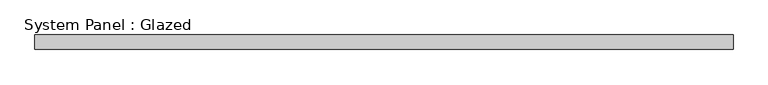
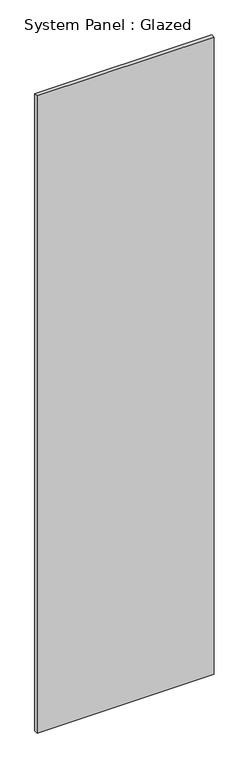
"""IFC4 building model written with IfcOpenShell, lengths in millimetres: plate geometry, System Panel : Glazed."""

import ifcopenshell
import ifcopenshell.guid

model = None  # the IFC model being written
_history = None  # IfcOwnerHistory: only IFC2X3 demands one
_inside = {}  # id of a spatial element -> (the spatial element, [elements in it])
_under = {}  # id of a project, library or spatial element -> (it, [spatial elements below it])
_declared = {}  # id of a project -> (the project, [libraries it declares])
_typed = {}  # id of a type object -> (the type object, [elements of that type])
_made_of = {}  # id of a material, layer set ... -> (it, [elements and type objects made of it])


def new_model(schema):
    """Start an empty IFC model of exactly this schema.

    Asked for "IFC4X3", IfcOpenShell would pick the latest addendum, in which some entities
    have other attributes; the version numbers below select the first issue.
    IFC2X3 requires an IfcOwnerHistory on every rooted entity: one is made here for all.
    """
    global model, _history
    if schema == "IFC4X3":
        model = ifcopenshell.file(schema_version=(4, 3, 0, 0))
    else:
        model = ifcopenshell.file(schema=schema)
    _inside.clear()
    _under.clear()
    _declared.clear()
    _typed.clear()
    _made_of.clear()
    _history = None
    if model.schema == "IFC2X3":
        org = make("IfcOrganization", Name="unknown")
        user = make(
            "IfcPersonAndOrganization",
            ThePerson=make("IfcPerson", FamilyName="unknown"),
            TheOrganization=org,
        )
        app = make(
            "IfcApplication",
            ApplicationDeveloper=org,
            Version="unknown",
            ApplicationFullName="unknown",
            ApplicationIdentifier="unknown",
        )
        _history = make(
            "IfcOwnerHistory",
            OwningUser=user,
            OwningApplication=app,
            ChangeAction="ADDED",
            CreationDate=0,
        )
    return model


def make(cls, **values):
    """One entity of the class cls with the attributes given. An attribute that is None is left unset."""
    return model.create_entity(
        cls, **{name: value for name, value in values.items() if value is not None}
    )


def rooted(cls, **values):
    """An entity with a GlobalId (a new one), such as an element, a storey or a relation."""
    return make(cls, GlobalId=ifcopenshell.guid.new(), OwnerHistory=_history, **values)


def si_unit(unit_type, name, prefix=None):
    """IfcSIUnit, for example si_unit("LENGTHUNIT", "METRE", prefix="MILLI")."""
    return make("IfcSIUnit", UnitType=unit_type, Prefix=prefix, Name=name)


def assignment(units):
    """IfcUnitAssignment: the units of a project."""
    return None if units is None else make("IfcUnitAssignment", Units=units)


def point(xyz):
    """IfcCartesianPoint."""
    return None if xyz is None else make("IfcCartesianPoint", Coordinates=xyz)


def direction(xyz):
    """IfcDirection."""
    return None if xyz is None else make("IfcDirection", DirectionRatios=xyz)


def frame(location, z_axis=None, x_axis=None):
    """IfcAxis2Placement3D, a coordinate frame: its origin and axes. An axis left out is left unset."""
    return make(
        "IfcAxis2Placement3D",
        Location=point(location),
        Axis=direction(z_axis),
        RefDirection=direction(x_axis),
    )


def origin():
    """The frame at (0, 0, 0) with its axes left unset."""
    return frame((0.0, 0.0, 0.0))


def origin_with_axes():
    """The frame at (0, 0, 0) with the z axis (0, 0, 1) and the x axis (1, 0, 0) written out."""
    return frame((0.0, 0.0, 0.0), z_axis=(0.0, 0.0, 1.0), x_axis=(1.0, 0.0, 0.0))


def place(relative_to, where):
    """IfcLocalPlacement: puts the frame where relative to a parent placement (None: the world)."""
    return make(
        "IfcLocalPlacement", PlacementRelTo=relative_to, RelativePlacement=where
    )


def context(
    kind, dimensions, precision=None, world=None, true_north=None, identifier=None
):
    """IfcGeometricRepresentationContext, for example the 3D "Model" context."""
    return make(
        "IfcGeometricRepresentationContext",
        ContextIdentifier=identifier,
        ContextType=kind,
        CoordinateSpaceDimension=dimensions,
        Precision=precision,
        WorldCoordinateSystem=world,
        TrueNorth=true_north,
    )


def project(units=None, contexts=None):
    """IfcProject with its units and contexts."""
    return rooted(
        "IfcProject",
        Name="project",
        RepresentationContexts=contexts,
        UnitsInContext=assignment(units),
    )


def spatial(cls, under=None, at=None, **own):
    """A site, building, storey or space (cls), placed at a placement, below another one or the project."""
    s = rooted(cls, ObjectPlacement=at, **own)
    if under is not None:
        _under.setdefault(under.id(), (under, []))[1].append(s)
    return s


def polyline(points):
    """IfcPolyline through the points."""
    return make("IfcPolyline", Points=[point(p) for p in points])


def outline(outer, holes=None, kind="AREA"):
    """IfcArbitraryClosedProfileDef: a profile drawn as a closed curve; with holes, ...WithVoids."""
    if holes is None:
        return make("IfcArbitraryClosedProfileDef", ProfileType=kind, OuterCurve=outer)
    return make(
        "IfcArbitraryProfileDefWithVoids",
        ProfileType=kind,
        OuterCurve=outer,
        InnerCurves=holes,
    )


def extrude(swept, where, along, depth):
    """IfcExtrudedAreaSolid: the profile swept, set in the frame where, extruded along a direction by depth."""
    return make(
        "IfcExtrudedAreaSolid",
        SweptArea=swept,
        Position=where,
        ExtrudedDirection=direction(along),
        Depth=depth,
    )


def shape(context_of_items, identifier, shape_type, items):
    """IfcShapeRepresentation: the items that make up one representation, for example the "Body"."""
    return make(
        "IfcShapeRepresentation",
        ContextOfItems=context_of_items,
        RepresentationIdentifier=identifier,
        RepresentationType=shape_type,
        Items=items,
    )


def source(mapping_origin, context_of_items, identifier, shape_type, items):
    """IfcRepresentationMap: a shape defined once, which mapped items show again and again."""
    return make(
        "IfcRepresentationMap",
        MappingOrigin=mapping_origin,
        MappedRepresentation=shape(context_of_items, identifier, shape_type, items),
    )


def transform(
    local_origin,
    x_axis=None,
    y_axis=None,
    z_axis=None,
    scale=None,
    scale2=None,
    scale3=None,
    uniform=True,
):
    """IfcCartesianTransformationOperator3D, or its non-uniform kind. x_axis, y_axis, z_axis: its Axis1, 2, 3."""
    if uniform:
        return make(
            "IfcCartesianTransformationOperator3D",
            Axis1=direction(x_axis),
            Axis2=direction(y_axis),
            LocalOrigin=point(local_origin),
            Scale=scale,
            Axis3=direction(z_axis),
        )
    return make(
        "IfcCartesianTransformationOperator3DnonUniform",
        Axis1=direction(x_axis),
        Axis2=direction(y_axis),
        LocalOrigin=point(local_origin),
        Scale=scale,
        Axis3=direction(z_axis),
        Scale2=scale2,
        Scale3=scale3,
    )


def mapped(mapping_source, mapping_target):
    """IfcMappedItem: shows the shape of a source again, moved by a transform."""
    return make(
        "IfcMappedItem", MappingSource=mapping_source, MappingTarget=mapping_target
    )


def made_of(thing, what):
    """Note that an element or type object is made of a material, layer set ...; save() writes the relation."""
    if what is not None:
        _made_of.setdefault(what.id(), (what, []))[1].append(thing)
    return thing


def element(
    cls,
    number,
    at=None,
    inside=None,
    cuts=None,
    type_object=None,
    material=None,
    context=None,
    identifier="Body",
    shape_type=None,
    held_by="IfcProductDefinitionShape",
    body=None,
    shapes=None,
    **own,
):
    """One element of the class cls, such as IfcWall. Its Tag is "e" and its number.

    at: its placement. inside: the storey or other place that contains it. cuts: it is an
    opening in that element (IfcRelVoidsElement). A single representation is given by context,
    identifier, shape_type and body (its items); several are given by shapes. held_by: the class
    of the entity that holds the representations. save() writes the other relations.
    """
    e = rooted(cls, Tag="e%d" % number, ObjectPlacement=at, **own)
    if body is not None:
        shapes = [shape(context, identifier, shape_type, body)]
    if shapes is not None:
        e.Representation = make(held_by, Representations=shapes)
    if inside is not None:
        _inside.setdefault(inside.id(), (inside, []))[1].append(e)
    if cuts is not None:
        rooted(
            "IfcRelVoidsElement", RelatingBuildingElement=cuts, RelatedOpeningElement=e
        )
    if type_object is not None:
        _typed.setdefault(type_object.id(), (type_object, []))[1].append(e)
    return made_of(e, material)


def aggregate(whole, parts):
    """IfcRelAggregates: a whole, such as a stair, and the parts it consists of."""
    return rooted("IfcRelAggregates", RelatingObject=whole, RelatedObjects=parts)


def save(model, path):
    """Write the relations noted so far, then the file.

    IfcRelAggregates (storeys below a building ...), IfcRelContainedInSpatialStructure (elements
    in a storey), IfcRelDefinesByType, IfcRelAssociatesMaterial and IfcRelDeclares: one each for
    every whole, place, type object, material and project.
    """
    for whole, parts in _under.values():
        aggregate(whole, parts)
    for where, things in _inside.values():
        rooted(
            "IfcRelContainedInSpatialStructure",
            RelatedElements=things,
            RelatingStructure=where,
        )
    for kind, things in _typed.values():
        rooted("IfcRelDefinesByType", RelatedObjects=things, RelatingType=kind)
    for what, things in _made_of.values():
        rooted("IfcRelAssociatesMaterial", RelatedObjects=things, RelatingMaterial=what)
    for by, libraries in _declared.values():
        rooted("IfcRelDeclares", RelatingContext=by, RelatedDefinitions=libraries)
    model.write(path)


def system_panel_glazed_31d10065(model_context):
    return source(origin(), model_context, "Body", "SweptSolid", [
        extrude(outline(polyline([(609.6, 19.05), (-609.6, 19.05), (-609.6, 44.45), (609.6, 44.45), (609.6, 19.05)])), origin_with_axes(), (0.0, 0.0, 1.0), 4629.15),
    ])


if __name__ == "__main__":
    model = new_model("IFC4")
    model_context = context("Model", 3, world=origin())
    ifc_project = project(units=[si_unit("LENGTHUNIT", "METRE", prefix="MILLI")], contexts=[model_context])
    site = spatial("IfcSite", under=ifc_project)
    building = spatial("IfcBuilding", under=site)
    placement = place(None, origin())
    system_panel_glazed_shape = system_panel_glazed_31d10065(model_context)
    element("IfcPlate", 1, ObjectType="System Panel : Glazed", at=placement, inside=building, context=model_context, shape_type="MappedRepresentation", body=[
        mapped(system_panel_glazed_shape, transform((0.0, 0.0, 0.0), x_axis=(1.0, 0.0, 0.0), y_axis=(0.0, 1.0, 0.0), z_axis=(0.0, 0.0, 1.0))),
    ])
    save(model, "model.ifc")

# Revit data of these elements
# Type "System Panel : Glazed"
#   Construction Type Id = "GSP4R"
#   Analytic Construction = "1/8 in Pilkington single glazing"
#   Visual Light Transmittance = 0.9
#   Solar Heat Gain Coefficient = 0.86
#   Heat Transfer Coefficient (U) = 1.18115 BTU/(h·ft²·°F)
#   Define Thermal Properties by = 1
# Element 1 (IfcPlate, "System Panel : Glazed")
#   Materials on its faces: "Glass"
# Materials
#   "Glass": class "Glass", colour RGB 0 128 192, transparency 0.75, Description = "Soda Lime Glass", Cost = 0
